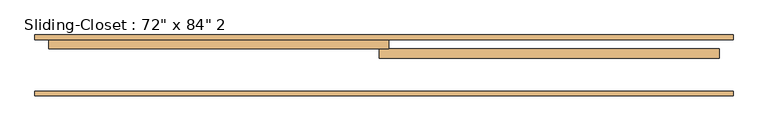
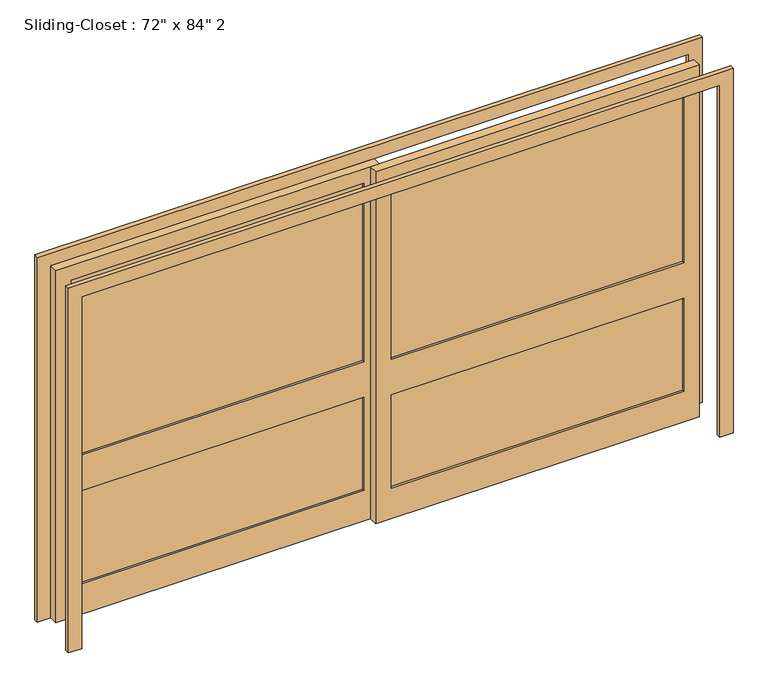
"""IFC4 building model written with IfcOpenShell, lengths in millimetres: door geometry."""

from ifc_helpers import new_model, si_unit, frame, origin, place, context, project, spatial, polyline, outline, extrude, source, transform, mapped, element, save


def door_976c1191(model_context):
    return source(origin(), model_context, "Body", "SweptSolid", [
        extrude(outline(polyline([(-63.5, 230.1875), (-1739.9, 230.1875), (-1739.9, 255.5875), (-63.5, 255.5875), (-63.5, 230.1875)])), frame((0.0, 0.0, 965.2), z_axis=(0.0, 0.0, 1.0), x_axis=(1.0, 0.0, 0.0)), (0.0, 0.0, 1.0), 1079.5),
        extrude(outline(polyline([(-63.5, 230.1875), (-1739.9, 230.1875), (-1739.9, 255.5875), (-63.5, 255.5875), (-63.5, 230.1875)])), frame((0.0, 0.0, 184.15), z_axis=(0.0, 0.0, 1.0), x_axis=(1.0, 0.0, 0.0)), (0.0, 0.0, 1.0), 565.15),
        extrude(outline(polyline([(63.5, 204.7875), (1739.9, 204.7875), (1739.9, 179.3875), (63.5, 179.3875), (63.5, 204.7875)])), frame((0.0, 0.0, 965.2), z_axis=(0.0, 0.0, 1.0), x_axis=(1.0, 0.0, 0.0)), (0.0, 0.0, 1.0), 1079.5),
        extrude(outline(polyline([(63.5, 204.7875), (1739.9, 204.7875), (1739.9, 179.3875), (63.5, 179.3875), (63.5, 204.7875)])), frame((0.0, 0.0, 184.15), z_axis=(0.0, 0.0, 1.0), x_axis=(1.0, 0.0, 0.0)), (0.0, 0.0, 1.0), 565.15),
        extrude(outline(polyline([(2133.6, 25.4), (2133.6, -1828.8), (0.0, -1828.8), (0.0, 25.4), (2133.6, 25.4)]), holes=[polyline([(184.15, -1739.9), (749.3, -1739.9), (749.3, -63.5), (184.15, -63.5), (184.15, -1739.9)]), polyline([(965.2, -1739.9), (2044.7, -1739.9), (2044.7, -63.5), (965.2, -63.5), (965.2, -1739.9)])]), frame((0.0, 217.4875, 0.0), z_axis=(0.0, 1.0, 0.0), x_axis=(0.0, 0.0, 1.0)), (0.0, 0.0, 1.0), 50.8),
        extrude(outline(polyline([(0.0, -1905.0), (0.0, -1828.8), (2133.6, -1828.8), (2133.6, 1828.8), (0.0, 1828.8), (0.0, 1905.0), (2209.8, 1905.0), (2209.8, -1905.0), (0.0, -1905.0)])), frame((0.0, -39.6875, 0.0), z_axis=(0.0, 1.0, 0.0), x_axis=(0.0, 0.0, 1.0)), (0.0, 0.0, 1.0), 25.4),
        extrude(outline(polyline([(0.0, 1905.0), (2209.8, 1905.0), (2209.8, -1905.0), (0.0, -1905.0), (0.0, -1828.8), (2133.6, -1828.8), (2133.6, 1828.8), (0.0, 1828.8), (0.0, 1905.0)])), frame((0.0, 268.2875, 0.0), z_axis=(0.0, 1.0, 0.0), x_axis=(0.0, 0.0, 1.0)), (0.0, 0.0, 1.0), 25.4),
        extrude(outline(polyline([(2133.6, -25.4), (0.0, -25.4), (0.0, 1828.8), (2133.6, 1828.8), (2133.6, -25.4)]), holes=[polyline([(965.2, 1739.9), (965.2, 63.5), (2044.7, 63.5), (2044.7, 1739.9), (965.2, 1739.9)]), polyline([(184.15, 1739.9), (184.15, 63.5), (749.3, 63.5), (749.3, 1739.9), (184.15, 1739.9)])]), frame((0.0, 166.6875, 0.0), z_axis=(0.0, 1.0, 0.0), x_axis=(0.0, 0.0, 1.0)), (0.0, 0.0, 1.0), 50.8),
    ])


if __name__ == "__main__":
    model = new_model("IFC4")
    model_context = context("Model", 3, world=origin())
    ifc_project = project(units=[si_unit("LENGTHUNIT", "METRE", prefix="MILLI")], contexts=[model_context])
    site = spatial("IfcSite", under=ifc_project)
    building = spatial("IfcBuilding", under=site)
    placement = place(None, origin())
    door_shape = door_976c1191(model_context)
    element("IfcDoor", 1, ObjectType="Sliding-Closet : 72\" x 84\" 2", at=placement, inside=building, context=model_context, shape_type="MappedRepresentation", body=[
        mapped(door_shape, transform((0.0, 0.0, 0.0), x_axis=(1.0, 0.0, 0.0), y_axis=(0.0, 1.0, 0.0), z_axis=(0.0, 0.0, 1.0))),
    ])
    save(model, "model.ifc")

# Revit data of these elements
# Type "Sliding-Closet : 72\" x 84\" 2"
#   Type Mark = "57"
#   Assembly Code = "C1020"
#   Thickness = 0' - 2"
#   Height = 7' - 0"
#   Trim Projection Ext = 0' - 1"
#   Trim Projection Int = 0' - 1"
#   Trim Width = 0' - 3"
#   Width = 12' - 0"
#   Door Material = Door - Panel
#   Frame Material = Door - Frame
#   Wall Closure = (empty or 0)
# Element 1 (IfcDoor, "Sliding-Closet : 72\" x 84\" 2")
#   Materials on its faces: "Door - Panel", "Door - Frame"
# Materials
#   "Door - Panel": class "Wood", colour RGB 227 170 128, transparency 0, Cost = 0
#   "Door - Frame": class "Miscellaneous", colour RGB 153 76 43, transparency 0, Cost = 0
